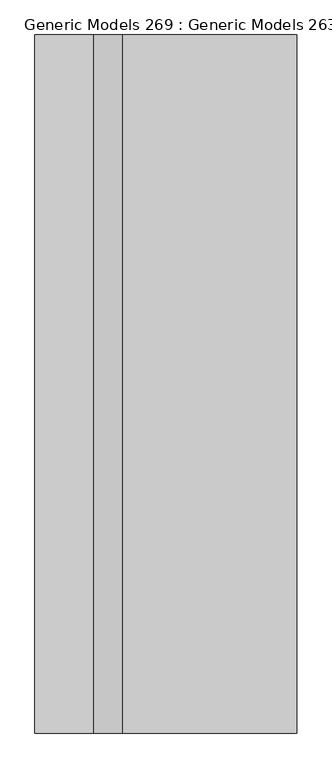
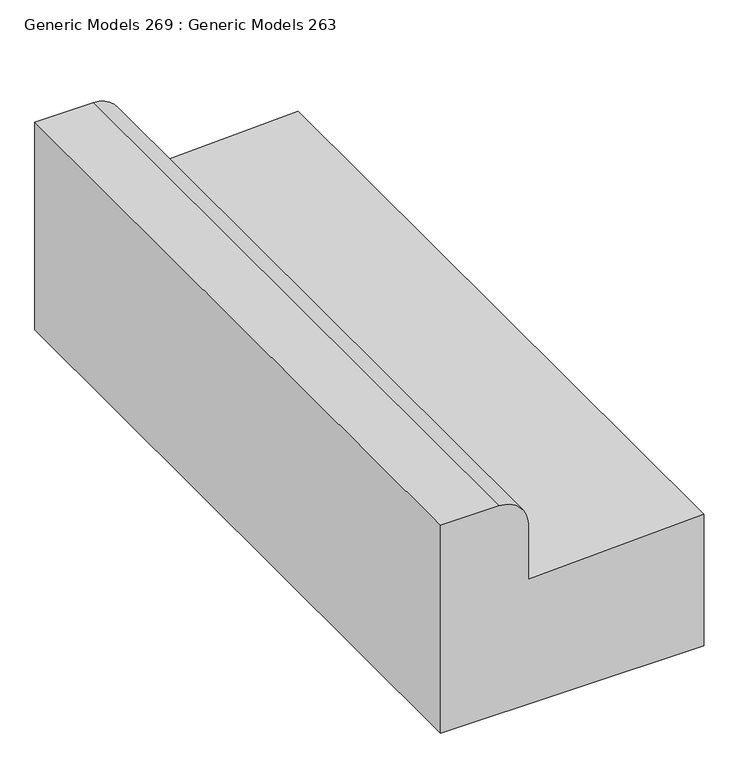
"""IFC4 building model written with IfcOpenShell, lengths in millimetres: proxy geometry, Generic Models 269 : Generic Models 263."""

import ifcopenshell
import ifcopenshell.guid

model = None  # the IFC model being written
_history = None  # IfcOwnerHistory: only IFC2X3 demands one
_inside = {}  # id of a spatial element -> (the spatial element, [elements in it])
_under = {}  # id of a project, library or spatial element -> (it, [spatial elements below it])
_declared = {}  # id of a project -> (the project, [libraries it declares])
_typed = {}  # id of a type object -> (the type object, [elements of that type])
_made_of = {}  # id of a material, layer set ... -> (it, [elements and type objects made of it])


def new_model(schema):
    """Start an empty IFC model of exactly this schema.

    Asked for "IFC4X3", IfcOpenShell would pick the latest addendum, in which some entities
    have other attributes; the version numbers below select the first issue.
    IFC2X3 requires an IfcOwnerHistory on every rooted entity: one is made here for all.
    """
    global model, _history
    if schema == "IFC4X3":
        model = ifcopenshell.file(schema_version=(4, 3, 0, 0))
    else:
        model = ifcopenshell.file(schema=schema)
    _inside.clear()
    _under.clear()
    _declared.clear()
    _typed.clear()
    _made_of.clear()
    _history = None
    if model.schema == "IFC2X3":
        org = make("IfcOrganization", Name="unknown")
        user = make(
            "IfcPersonAndOrganization",
            ThePerson=make("IfcPerson", FamilyName="unknown"),
            TheOrganization=org,
        )
        app = make(
            "IfcApplication",
            ApplicationDeveloper=org,
            Version="unknown",
            ApplicationFullName="unknown",
            ApplicationIdentifier="unknown",
        )
        _history = make(
            "IfcOwnerHistory",
            OwningUser=user,
            OwningApplication=app,
            ChangeAction="ADDED",
            CreationDate=0,
        )
    return model


def make(cls, **values):
    """One entity of the class cls with the attributes given. An attribute that is None is left unset."""
    return model.create_entity(
        cls, **{name: value for name, value in values.items() if value is not None}
    )


def rooted(cls, **values):
    """An entity with a GlobalId (a new one), such as an element, a storey or a relation."""
    return make(cls, GlobalId=ifcopenshell.guid.new(), OwnerHistory=_history, **values)


def si_unit(unit_type, name, prefix=None):
    """IfcSIUnit, for example si_unit("LENGTHUNIT", "METRE", prefix="MILLI")."""
    return make("IfcSIUnit", UnitType=unit_type, Prefix=prefix, Name=name)


def assignment(units):
    """IfcUnitAssignment: the units of a project."""
    return None if units is None else make("IfcUnitAssignment", Units=units)


def point(xyz):
    """IfcCartesianPoint."""
    return None if xyz is None else make("IfcCartesianPoint", Coordinates=xyz)


def direction(xyz):
    """IfcDirection."""
    return None if xyz is None else make("IfcDirection", DirectionRatios=xyz)


def frame(location, z_axis=None, x_axis=None):
    """IfcAxis2Placement3D, a coordinate frame: its origin and axes. An axis left out is left unset."""
    return make(
        "IfcAxis2Placement3D",
        Location=point(location),
        Axis=direction(z_axis),
        RefDirection=direction(x_axis),
    )


def frame_2d(location, x_axis=None):
    """IfcAxis2Placement2D, a coordinate frame in the plane: its origin and x axis."""
    return make(
        "IfcAxis2Placement2D", Location=point(location), RefDirection=direction(x_axis)
    )


def origin():
    """The frame at (0, 0, 0) with its axes left unset."""
    return frame((0.0, 0.0, 0.0))


def place(relative_to, where):
    """IfcLocalPlacement: puts the frame where relative to a parent placement (None: the world)."""
    return make(
        "IfcLocalPlacement", PlacementRelTo=relative_to, RelativePlacement=where
    )


def context(
    kind, dimensions, precision=None, world=None, true_north=None, identifier=None
):
    """IfcGeometricRepresentationContext, for example the 3D "Model" context."""
    return make(
        "IfcGeometricRepresentationContext",
        ContextIdentifier=identifier,
        ContextType=kind,
        CoordinateSpaceDimension=dimensions,
        Precision=precision,
        WorldCoordinateSystem=world,
        TrueNorth=true_north,
    )


def project(units=None, contexts=None):
    """IfcProject with its units and contexts."""
    return rooted(
        "IfcProject",
        Name="project",
        RepresentationContexts=contexts,
        UnitsInContext=assignment(units),
    )


def spatial(cls, under=None, at=None, **own):
    """A site, building, storey or space (cls), placed at a placement, below another one or the project."""
    s = rooted(cls, ObjectPlacement=at, **own)
    if under is not None:
        _under.setdefault(under.id(), (under, []))[1].append(s)
    return s


def polyline(points):
    """IfcPolyline through the points."""
    return make("IfcPolyline", Points=[point(p) for p in points])


def circle_curve(where, radius):
    """IfcCircle in the frame where."""
    return make("IfcCircle", Position=where, Radius=radius)


def trimmed(basis, trim1, trim2, sense, master):
    """IfcTrimmedCurve: the piece of a basis curve between two trims."""
    return make(
        "IfcTrimmedCurve",
        BasisCurve=basis,
        Trim1=trim1,
        Trim2=trim2,
        SenseAgreement=sense,
        MasterRepresentation=master,
    )


def segment(curve, same_sense, transition):
    """IfcCompositeCurveSegment."""
    return make(
        "IfcCompositeCurveSegment",
        Transition=transition,
        SameSense=same_sense,
        ParentCurve=curve,
    )


def composite_curve(segments, self_intersect=None):
    """IfcCompositeCurve: segments joined end to end."""
    return make("IfcCompositeCurve", Segments=segments, SelfIntersect=self_intersect)


def outline(outer, holes=None, kind="AREA"):
    """IfcArbitraryClosedProfileDef: a profile drawn as a closed curve; with holes, ...WithVoids."""
    if holes is None:
        return make("IfcArbitraryClosedProfileDef", ProfileType=kind, OuterCurve=outer)
    return make(
        "IfcArbitraryProfileDefWithVoids",
        ProfileType=kind,
        OuterCurve=outer,
        InnerCurves=holes,
    )


def extrude(swept, where, along, depth):
    """IfcExtrudedAreaSolid: the profile swept, set in the frame where, extruded along a direction by depth."""
    return make(
        "IfcExtrudedAreaSolid",
        SweptArea=swept,
        Position=where,
        ExtrudedDirection=direction(along),
        Depth=depth,
    )


def shape(context_of_items, identifier, shape_type, items):
    """IfcShapeRepresentation: the items that make up one representation, for example the "Body"."""
    return make(
        "IfcShapeRepresentation",
        ContextOfItems=context_of_items,
        RepresentationIdentifier=identifier,
        RepresentationType=shape_type,
        Items=items,
    )


def source(mapping_origin, context_of_items, identifier, shape_type, items):
    """IfcRepresentationMap: a shape defined once, which mapped items show again and again."""
    return make(
        "IfcRepresentationMap",
        MappingOrigin=mapping_origin,
        MappedRepresentation=shape(context_of_items, identifier, shape_type, items),
    )


def transform(
    local_origin,
    x_axis=None,
    y_axis=None,
    z_axis=None,
    scale=None,
    scale2=None,
    scale3=None,
    uniform=True,
):
    """IfcCartesianTransformationOperator3D, or its non-uniform kind. x_axis, y_axis, z_axis: its Axis1, 2, 3."""
    if uniform:
        return make(
            "IfcCartesianTransformationOperator3D",
            Axis1=direction(x_axis),
            Axis2=direction(y_axis),
            LocalOrigin=point(local_origin),
            Scale=scale,
            Axis3=direction(z_axis),
        )
    return make(
        "IfcCartesianTransformationOperator3DnonUniform",
        Axis1=direction(x_axis),
        Axis2=direction(y_axis),
        LocalOrigin=point(local_origin),
        Scale=scale,
        Axis3=direction(z_axis),
        Scale2=scale2,
        Scale3=scale3,
    )


def mapped(mapping_source, mapping_target):
    """IfcMappedItem: shows the shape of a source again, moved by a transform."""
    return make(
        "IfcMappedItem", MappingSource=mapping_source, MappingTarget=mapping_target
    )


def made_of(thing, what):
    """Note that an element or type object is made of a material, layer set ...; save() writes the relation."""
    if what is not None:
        _made_of.setdefault(what.id(), (what, []))[1].append(thing)
    return thing


def element(
    cls,
    number,
    at=None,
    inside=None,
    cuts=None,
    type_object=None,
    material=None,
    context=None,
    identifier="Body",
    shape_type=None,
    held_by="IfcProductDefinitionShape",
    body=None,
    shapes=None,
    **own,
):
    """One element of the class cls, such as IfcWall. Its Tag is "e" and its number.

    at: its placement. inside: the storey or other place that contains it. cuts: it is an
    opening in that element (IfcRelVoidsElement). A single representation is given by context,
    identifier, shape_type and body (its items); several are given by shapes. held_by: the class
    of the entity that holds the representations. save() writes the other relations.
    """
    e = rooted(cls, Tag="e%d" % number, ObjectPlacement=at, **own)
    if body is not None:
        shapes = [shape(context, identifier, shape_type, body)]
    if shapes is not None:
        e.Representation = make(held_by, Representations=shapes)
    if inside is not None:
        _inside.setdefault(inside.id(), (inside, []))[1].append(e)
    if cuts is not None:
        rooted(
            "IfcRelVoidsElement", RelatingBuildingElement=cuts, RelatedOpeningElement=e
        )
    if type_object is not None:
        _typed.setdefault(type_object.id(), (type_object, []))[1].append(e)
    return made_of(e, material)


def aggregate(whole, parts):
    """IfcRelAggregates: a whole, such as a stair, and the parts it consists of."""
    return rooted("IfcRelAggregates", RelatingObject=whole, RelatedObjects=parts)


def save(model, path):
    """Write the relations noted so far, then the file.

    IfcRelAggregates (storeys below a building ...), IfcRelContainedInSpatialStructure (elements
    in a storey), IfcRelDefinesByType, IfcRelAssociatesMaterial and IfcRelDeclares: one each for
    every whole, place, type object, material and project.
    """
    for whole, parts in _under.values():
        aggregate(whole, parts)
    for where, things in _inside.values():
        rooted(
            "IfcRelContainedInSpatialStructure",
            RelatedElements=things,
            RelatingStructure=where,
        )
    for kind, things in _typed.values():
        rooted("IfcRelDefinesByType", RelatedObjects=things, RelatingType=kind)
    for what, things in _made_of.values():
        rooted("IfcRelAssociatesMaterial", RelatedObjects=things, RelatingMaterial=what)
    for by, libraries in _declared.values():
        rooted("IfcRelDeclares", RelatingContext=by, RelatedDefinitions=libraries)
    model.write(path)


def generic_models_269_generic_models_263_66db3b1b(model_context):
    return source(origin(), model_context, "Body", "SweptSolid", [
        extrude(outline(composite_curve([segment(polyline([(0.0, 60591.9797726), (0.0, 60490.3797726), (-381.0, 60490.3797726), (-381.0, 60947.5797726), (-139.7, 60947.5797726), (-152.4, 60642.7797726), (-50.8, 60642.7797726)]), True, "CONTINUOUS"), segment(trimmed(circle_curve(frame_2d((-50.8, 60591.9797726)), 50.8), [point((-50.8, 60642.7797726))], [point((0.0, 60591.9797726))], False, "CARTESIAN"), True, "CONTINUOUS")], self_intersect=False)), frame((0.0, -94.4486541, 0.0), z_axis=(0.0, 1.0, 0.0), x_axis=(0.0, 0.0, 1.0)), (0.0, 0.0, 1.0), 1219.2),
    ])


if __name__ == "__main__":
    model = new_model("IFC4")
    model_context = context("Model", 3, world=origin())
    ifc_project = project(units=[si_unit("LENGTHUNIT", "METRE", prefix="MILLI")], contexts=[model_context])
    site = spatial("IfcSite", under=ifc_project)
    building = spatial("IfcBuilding", under=site)
    placement = place(None, origin())
    generic_models_269_generic_models_263_shape = generic_models_269_generic_models_263_66db3b1b(model_context)
    element("IfcBuildingElementProxy", 1, Name="Generic Models 269 : Generic Models 263", ObjectType="Generic Models 269 : Generic Models 263", at=placement, inside=building, context=model_context, shape_type="MappedRepresentation", body=[
        mapped(generic_models_269_generic_models_263_shape, transform((0.0, 0.0, 0.0), x_axis=(1.0, 0.0, 0.0), y_axis=(0.0, 1.0, 0.0), z_axis=(0.0, 0.0, 1.0))),
    ])
    save(model, "model.ifc")

# Revit data of these elements
# Element 1 (IfcBuildingElementProxy, "Generic Models 269 : Generic Models 263")
#   Materials on its faces: "CONCRETE CURB"
# Materials
#   "CONCRETE CURB": class "Concrete", colour RGB 191 191 191, transparency 0, Description = "Cast-in-place concrete", Cost = 0
